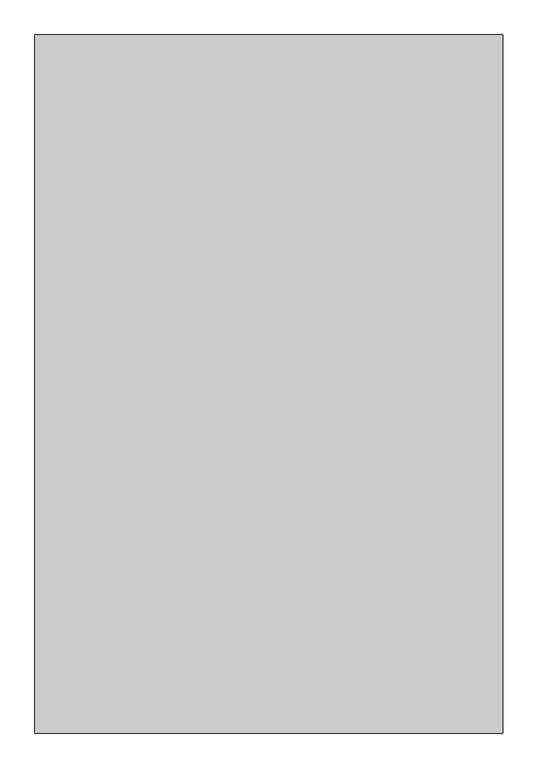
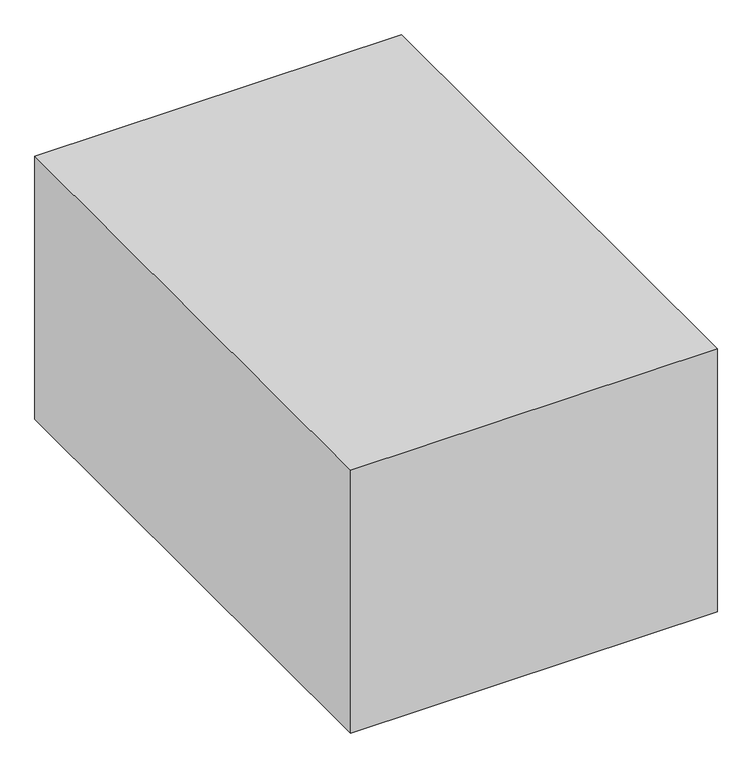
"""IFC4 building model written with IfcOpenShell, lengths in millimetres: proxy geometry, 0_3d."""

from ifc_helpers import new_model, si_unit, origin, origin_with_axes, place, context, project, spatial, polyline, outline, extrude, source, transform, mapped, element, save


def generic_models_1baf5907(model_context):
    return source(origin(), model_context, "Body", "SweptSolid", [
        extrude(outline(polyline([(3800.0, 0.0), (0.0, 0.0), (0.0, 5670.0), (3800.0, 5670.0), (3800.0, 0.0)])), origin_with_axes(), (0.0, 0.0, 1.0), 2880.0),
    ])


if __name__ == "__main__":
    model = new_model("IFC4")
    model_context = context("Model", 3, world=origin())
    ifc_project = project(units=[si_unit("LENGTHUNIT", "METRE", prefix="MILLI")], contexts=[model_context])
    site = spatial("IfcSite", under=ifc_project)
    building = spatial("IfcBuilding", under=site)
    placement = place(None, origin())
    generic_models_shape = generic_models_1baf5907(model_context)
    element("IfcBuildingElementProxy", 1, Name="0_3d", ObjectType="0_3d", at=placement, inside=building, context=model_context, shape_type="MappedRepresentation", body=[
        mapped(generic_models_shape, transform((0.0, 0.0, 0.0), x_axis=(1.0, 0.0, 0.0), y_axis=(0.0, 1.0, 0.0), z_axis=(0.0, 0.0, 1.0))),
    ])
    save(model, "model.ifc")

# Revit data of these elements
# Element 1 (IfcBuildingElementProxy, "0_3d")
#   Materials on its faces: "*1"
# Materials
#   "*1": class "Unassigned", colour RGB 175 175 175, transparency 0
